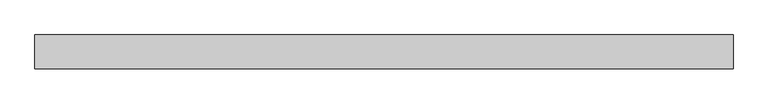
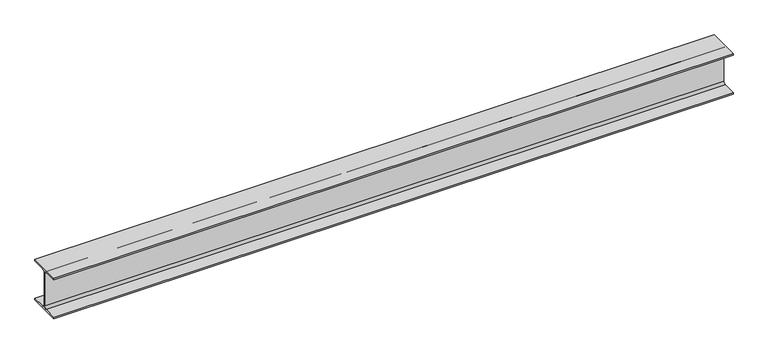
"""IFC4 building model written with IfcOpenShell, lengths in millimetres: beam geometry, 0912_Steel Framing_H-KSD3502 : H_SB_ASB_H-390x300x10x16."""

from ifc_helpers import new_model, si_unit, point, frame, frame_2d, origin, place, context, project, spatial, polyline, circle_curve, trimmed, segment, composite_curve, outline, extrude, source, transform, mapped, element, save


def beam_051c4779(model_context):
    return source(origin(), model_context, "Body", "SweptSolid", [
        extrude(outline(composite_curve([segment(polyline([(150.0, -179.0), (150.0, -195.0), (-150.0, -195.0), (-150.0, -179.0), (-27.0, -179.0)]), True, "CONTINUOUS"), segment(trimmed(circle_curve(frame_2d((-27.0, -157.0)), 22.0), [point((-27.0, -179.0))], [point((-5.0, -157.0))], True, "CARTESIAN"), True, "CONTINUOUS"), segment(polyline([(-5.0, -157.0), (-5.0, 157.0)]), True, "CONTINUOUS"), segment(trimmed(circle_curve(frame_2d((-27.0, 157.0)), 22.0), [point((-5.0, 157.0))], [point((-27.0, 179.0))], True, "CARTESIAN"), True, "CONTINUOUS"), segment(polyline([(-27.0, 179.0), (-150.0, 179.0), (-150.0, 195.0), (150.0, 195.0), (150.0, 179.0), (27.0, 179.0)]), True, "CONTINUOUS"), segment(trimmed(circle_curve(frame_2d((27.0, 157.0)), 22.0), [point((27.0, 179.0))], [point((5.0, 157.0))], True, "CARTESIAN"), True, "CONTINUOUS"), segment(polyline([(5.0, 157.0), (5.0, -157.0)]), True, "CONTINUOUS"), segment(trimmed(circle_curve(frame_2d((27.0, -157.0)), 22.0), [point((5.0, -157.0))], [point((27.0, -179.0))], True, "CARTESIAN"), True, "CONTINUOUS"), segment(polyline([(27.0, -179.0), (150.0, -179.0)]), True, "CONTINUOUS")], self_intersect=False)), frame((-3087.3, 0.0, 0.0), z_axis=(1.0, 0.0, 0.0), x_axis=(0.0, 1.0, 0.0)), (0.0, 0.0, 1.0), 6174.6),
    ])


if __name__ == "__main__":
    model = new_model("IFC4")
    model_context = context("Model", 3, world=origin())
    ifc_project = project(units=[si_unit("LENGTHUNIT", "METRE", prefix="MILLI")], contexts=[model_context])
    site = spatial("IfcSite", under=ifc_project)
    building = spatial("IfcBuilding", under=site)
    placement = place(None, origin())
    beam_shape = beam_051c4779(model_context)
    element("IfcBeam", 1, ObjectType="0912_Steel Framing_H-KSD3502 : H_SB_ASB_H-390x300x10x16", at=placement, inside=building, context=model_context, shape_type="MappedRepresentation", body=[
        mapped(beam_shape, transform((0.0, 0.0, 0.0), x_axis=(1.0, 0.0, 0.0), y_axis=(0.0, 1.0, 0.0), z_axis=(0.0, 0.0, 1.0))),
    ])
    save(model, "model.ifc")

# Revit data of these elements
# Type "0912_Steel Framing_H-KSD3502 : H_SB_ASB_H-390x300x10x16"
#   H_WM Code_1 = "S01AA001-00001 | Main Steel Structure Fabrication Work | Shelter/Building | Heavy Steel - Standard (Weight≥90KG/M) | Material: (   )"
#   H_WM Code_2 = "S03AA027-00001 | Main Steel Structure Erection Work | Shelter/Building | Heavy Steel (Weight≥90KG/M) | Material: (   )"
#   H_WM Code_3 = "S01AA010-00001 | Main Steel Structure Fabrication Work | Shelter/Building | Steel Painting/Coating | for Non-Fireproofed Steel Surface, Surface Preparation, Primer, Second & Final Coat | Material: (   )"
#   H_Q'ty Cal Type Tag = "SB-Q2"
#   Width = 30.0 cm
#   Web Thickness = 1.0 cm
#   Web Fillet = 2.2 cm
#   Warping Constant = 2520000.0 cm⁶
#   W = 0
#   Torsional Moment of Inertia = 94.3867 cm⁴
#   Section Area = 136.0 cm²
#   Plastic Modulus weak axis = 733.0 cm³
#   Plastic Modulus strong axis = 2190.0 cm³
#   Perimeter = 1.92 m²/m
#   Nominal Weight = 107.00 kgf/m
#   Moment of Inertia weak axis = 7210.00 cm⁴
#   Moment of Inertia strong axis = 38700.00 cm⁴
#   Height = 39.0 cm
#   Flange Thickness = 1.6 cm
#   Elastic Modulus weak axis = 481.0 cm³
#   Elastic Modulus strong axis = 1980.0 cm³
#   Centroid Vertical = 19.5 cm
#   Centroid Horizontal = 15.0 cm
#   Ix = 387000000
#   Length [instance default] = 1.5240 m
#   Zx = 2190000
#   b = 0.3000 m
#   h = 0.3900 m
#   r = 0.0220 m
#   s = 0.0100 m
#   t = 0.0160 m
#   A = 0.0136 m²
#   Structural Material [instance default] = Steel, 45-345
#   Assembly Code = ""
# Element 1 (IfcBeam, "0912_Steel Framing_H-KSD3502 : H_SB_ASB_H-390x300x10x16")
#   Structural Material = none
# Materials
#   "Steel, 45-345": class "Metal", colour RGB 189 187 185, transparency 0, Description = "Steel 345 MPa", Cost = 0
